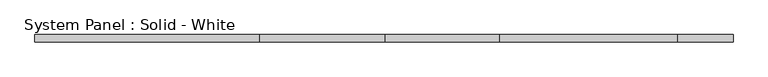
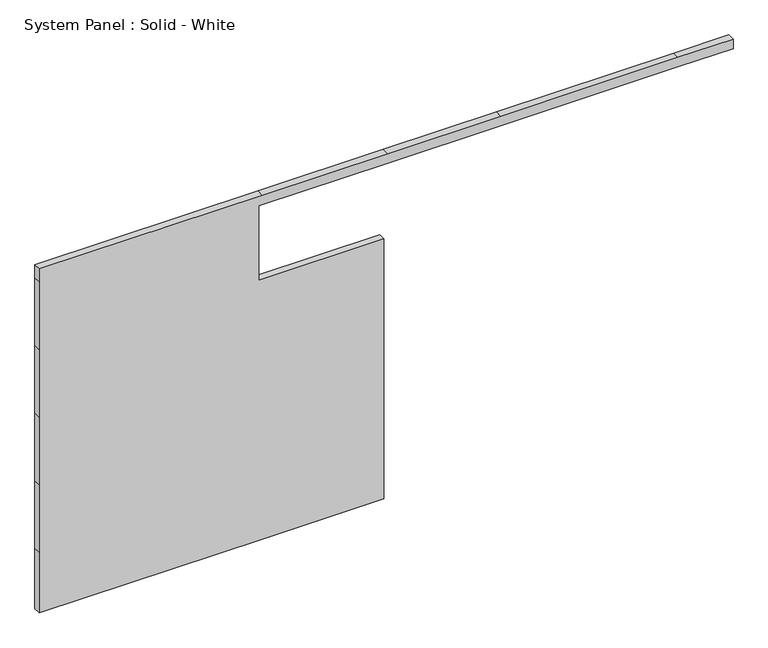
"""IFC4 building model written with IfcOpenShell, lengths in millimetres: plate geometry, System Panel : Solid - White."""

from ifc_helpers import new_model, si_unit, frame, origin, place, context, project, spatial, polyline, outline, extrude, source, transform, mapped, element, save


def system_panel_solid_white_a9903a75(model_context):
    return source(origin(), model_context, "Body", "SweptSolid", [
        extrude(outline(polyline([(0.0, -2959.1), (0.0, -1055.3257062), (0.0, -19.05), (546.1, -19.05), (1155.7, -19.05), (1765.3, -19.05), (2343.15, -19.05), (2343.15, -1087.0757062), (3016.25, -1087.0757062), (3016.25, 12.7), (3016.25, 979.1257062), (3016.25, 2489.2), (3016.25, 2959.1), (3101.9419949, 2959.1), (3101.9419949, 2489.2), (3101.9419949, 979.1257062), (3101.9419949, 12.7), (3101.9419949, -1055.3257062), (3101.9419949, -2959.1), (2984.5, -2959.1), (2374.9, -2959.1), (1765.3, -2959.1), (1155.7, -2959.1), (546.1, -2959.1), (0.0, -2959.1)])), frame((0.0, -44.45, 0.0), z_axis=(0.0, 1.0, 0.0), x_axis=(0.0, 0.0, 1.0)), (0.0, 0.0, 1.0), 63.5),
    ])


if __name__ == "__main__":
    model = new_model("IFC4")
    model_context = context("Model", 3, world=origin())
    ifc_project = project(units=[si_unit("LENGTHUNIT", "METRE", prefix="MILLI")], contexts=[model_context])
    site = spatial("IfcSite", under=ifc_project)
    building = spatial("IfcBuilding", under=site)
    placement = place(None, origin())
    system_panel_solid_white_shape = system_panel_solid_white_a9903a75(model_context)
    element("IfcPlate", 1, ObjectType="System Panel : Solid - White", at=placement, inside=building, context=model_context, shape_type="MappedRepresentation", body=[
        mapped(system_panel_solid_white_shape, transform((0.0, 0.0, 0.0), x_axis=(1.0, 0.0, 0.0), y_axis=(0.0, 1.0, 0.0), z_axis=(0.0, 0.0, 1.0))),
    ])
    save(model, "model.ifc")

# Revit data of these elements
# Element 1 (IfcPlate, "System Panel : Solid - White")
#   Materials on its faces: "White Panel"
# Materials
#   "White Panel": class "Unassigned", colour RGB 255 255 255, transparency 0
